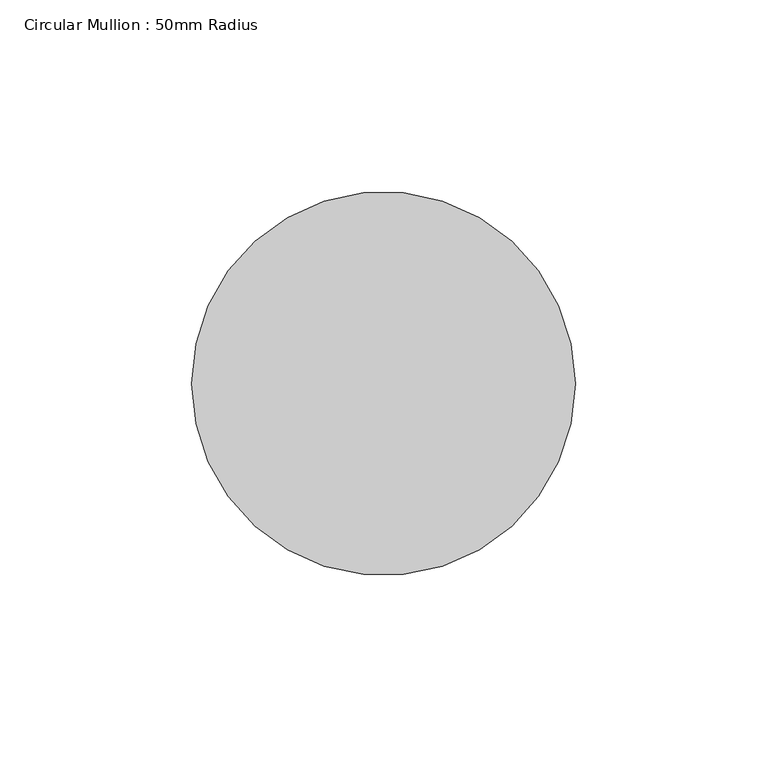
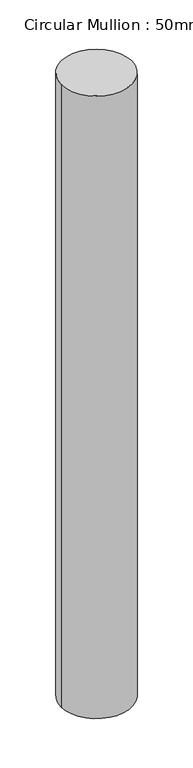
"""IFC4 building model written with IfcOpenShell, lengths in millimetres: member geometry, Circular Mullion : 50mm Radius."""

import ifcopenshell
import ifcopenshell.guid

model = None  # the IFC model being written
_history = None  # IfcOwnerHistory: only IFC2X3 demands one
_inside = {}  # id of a spatial element -> (the spatial element, [elements in it])
_under = {}  # id of a project, library or spatial element -> (it, [spatial elements below it])
_declared = {}  # id of a project -> (the project, [libraries it declares])
_typed = {}  # id of a type object -> (the type object, [elements of that type])
_made_of = {}  # id of a material, layer set ... -> (it, [elements and type objects made of it])


def new_model(schema):
    """Start an empty IFC model of exactly this schema.

    Asked for "IFC4X3", IfcOpenShell would pick the latest addendum, in which some entities
    have other attributes; the version numbers below select the first issue.
    IFC2X3 requires an IfcOwnerHistory on every rooted entity: one is made here for all.
    """
    global model, _history
    if schema == "IFC4X3":
        model = ifcopenshell.file(schema_version=(4, 3, 0, 0))
    else:
        model = ifcopenshell.file(schema=schema)
    _inside.clear()
    _under.clear()
    _declared.clear()
    _typed.clear()
    _made_of.clear()
    _history = None
    if model.schema == "IFC2X3":
        org = make("IfcOrganization", Name="unknown")
        user = make(
            "IfcPersonAndOrganization",
            ThePerson=make("IfcPerson", FamilyName="unknown"),
            TheOrganization=org,
        )
        app = make(
            "IfcApplication",
            ApplicationDeveloper=org,
            Version="unknown",
            ApplicationFullName="unknown",
            ApplicationIdentifier="unknown",
        )
        _history = make(
            "IfcOwnerHistory",
            OwningUser=user,
            OwningApplication=app,
            ChangeAction="ADDED",
            CreationDate=0,
        )
    return model


def make(cls, **values):
    """One entity of the class cls with the attributes given. An attribute that is None is left unset."""
    return model.create_entity(
        cls, **{name: value for name, value in values.items() if value is not None}
    )


def rooted(cls, **values):
    """An entity with a GlobalId (a new one), such as an element, a storey or a relation."""
    return make(cls, GlobalId=ifcopenshell.guid.new(), OwnerHistory=_history, **values)


def si_unit(unit_type, name, prefix=None):
    """IfcSIUnit, for example si_unit("LENGTHUNIT", "METRE", prefix="MILLI")."""
    return make("IfcSIUnit", UnitType=unit_type, Prefix=prefix, Name=name)


def assignment(units):
    """IfcUnitAssignment: the units of a project."""
    return None if units is None else make("IfcUnitAssignment", Units=units)


def point(xyz):
    """IfcCartesianPoint."""
    return None if xyz is None else make("IfcCartesianPoint", Coordinates=xyz)


def direction(xyz):
    """IfcDirection."""
    return None if xyz is None else make("IfcDirection", DirectionRatios=xyz)


def frame(location, z_axis=None, x_axis=None):
    """IfcAxis2Placement3D, a coordinate frame: its origin and axes. An axis left out is left unset."""
    return make(
        "IfcAxis2Placement3D",
        Location=point(location),
        Axis=direction(z_axis),
        RefDirection=direction(x_axis),
    )


def frame_2d(location, x_axis=None):
    """IfcAxis2Placement2D, a coordinate frame in the plane: its origin and x axis."""
    return make(
        "IfcAxis2Placement2D", Location=point(location), RefDirection=direction(x_axis)
    )


def origin():
    """The frame at (0, 0, 0) with its axes left unset."""
    return frame((0.0, 0.0, 0.0))


def origin_2d():
    """The frame at (0, 0) in the plane with its x axis left unset."""
    return frame_2d((0.0, 0.0))


def place(relative_to, where):
    """IfcLocalPlacement: puts the frame where relative to a parent placement (None: the world)."""
    return make(
        "IfcLocalPlacement", PlacementRelTo=relative_to, RelativePlacement=where
    )


def context(
    kind, dimensions, precision=None, world=None, true_north=None, identifier=None
):
    """IfcGeometricRepresentationContext, for example the 3D "Model" context."""
    return make(
        "IfcGeometricRepresentationContext",
        ContextIdentifier=identifier,
        ContextType=kind,
        CoordinateSpaceDimension=dimensions,
        Precision=precision,
        WorldCoordinateSystem=world,
        TrueNorth=true_north,
    )


def project(units=None, contexts=None):
    """IfcProject with its units and contexts."""
    return rooted(
        "IfcProject",
        Name="project",
        RepresentationContexts=contexts,
        UnitsInContext=assignment(units),
    )


def spatial(cls, under=None, at=None, **own):
    """A site, building, storey or space (cls), placed at a placement, below another one or the project."""
    s = rooted(cls, ObjectPlacement=at, **own)
    if under is not None:
        _under.setdefault(under.id(), (under, []))[1].append(s)
    return s


def circle_curve(where, radius):
    """IfcCircle in the frame where."""
    return make("IfcCircle", Position=where, Radius=radius)


def trimmed(basis, trim1, trim2, sense, master):
    """IfcTrimmedCurve: the piece of a basis curve between two trims."""
    return make(
        "IfcTrimmedCurve",
        BasisCurve=basis,
        Trim1=trim1,
        Trim2=trim2,
        SenseAgreement=sense,
        MasterRepresentation=master,
    )


def segment(curve, same_sense, transition):
    """IfcCompositeCurveSegment."""
    return make(
        "IfcCompositeCurveSegment",
        Transition=transition,
        SameSense=same_sense,
        ParentCurve=curve,
    )


def composite_curve(segments, self_intersect=None):
    """IfcCompositeCurve: segments joined end to end."""
    return make("IfcCompositeCurve", Segments=segments, SelfIntersect=self_intersect)


def outline(outer, holes=None, kind="AREA"):
    """IfcArbitraryClosedProfileDef: a profile drawn as a closed curve; with holes, ...WithVoids."""
    if holes is None:
        return make("IfcArbitraryClosedProfileDef", ProfileType=kind, OuterCurve=outer)
    return make(
        "IfcArbitraryProfileDefWithVoids",
        ProfileType=kind,
        OuterCurve=outer,
        InnerCurves=holes,
    )


def extrude(swept, where, along, depth):
    """IfcExtrudedAreaSolid: the profile swept, set in the frame where, extruded along a direction by depth."""
    return make(
        "IfcExtrudedAreaSolid",
        SweptArea=swept,
        Position=where,
        ExtrudedDirection=direction(along),
        Depth=depth,
    )


def shape(context_of_items, identifier, shape_type, items):
    """IfcShapeRepresentation: the items that make up one representation, for example the "Body"."""
    return make(
        "IfcShapeRepresentation",
        ContextOfItems=context_of_items,
        RepresentationIdentifier=identifier,
        RepresentationType=shape_type,
        Items=items,
    )


def source(mapping_origin, context_of_items, identifier, shape_type, items):
    """IfcRepresentationMap: a shape defined once, which mapped items show again and again."""
    return make(
        "IfcRepresentationMap",
        MappingOrigin=mapping_origin,
        MappedRepresentation=shape(context_of_items, identifier, shape_type, items),
    )


def transform(
    local_origin,
    x_axis=None,
    y_axis=None,
    z_axis=None,
    scale=None,
    scale2=None,
    scale3=None,
    uniform=True,
):
    """IfcCartesianTransformationOperator3D, or its non-uniform kind. x_axis, y_axis, z_axis: its Axis1, 2, 3."""
    if uniform:
        return make(
            "IfcCartesianTransformationOperator3D",
            Axis1=direction(x_axis),
            Axis2=direction(y_axis),
            LocalOrigin=point(local_origin),
            Scale=scale,
            Axis3=direction(z_axis),
        )
    return make(
        "IfcCartesianTransformationOperator3DnonUniform",
        Axis1=direction(x_axis),
        Axis2=direction(y_axis),
        LocalOrigin=point(local_origin),
        Scale=scale,
        Axis3=direction(z_axis),
        Scale2=scale2,
        Scale3=scale3,
    )


def mapped(mapping_source, mapping_target):
    """IfcMappedItem: shows the shape of a source again, moved by a transform."""
    return make(
        "IfcMappedItem", MappingSource=mapping_source, MappingTarget=mapping_target
    )


def made_of(thing, what):
    """Note that an element or type object is made of a material, layer set ...; save() writes the relation."""
    if what is not None:
        _made_of.setdefault(what.id(), (what, []))[1].append(thing)
    return thing


def element(
    cls,
    number,
    at=None,
    inside=None,
    cuts=None,
    type_object=None,
    material=None,
    context=None,
    identifier="Body",
    shape_type=None,
    held_by="IfcProductDefinitionShape",
    body=None,
    shapes=None,
    **own,
):
    """One element of the class cls, such as IfcWall. Its Tag is "e" and its number.

    at: its placement. inside: the storey or other place that contains it. cuts: it is an
    opening in that element (IfcRelVoidsElement). A single representation is given by context,
    identifier, shape_type and body (its items); several are given by shapes. held_by: the class
    of the entity that holds the representations. save() writes the other relations.
    """
    e = rooted(cls, Tag="e%d" % number, ObjectPlacement=at, **own)
    if body is not None:
        shapes = [shape(context, identifier, shape_type, body)]
    if shapes is not None:
        e.Representation = make(held_by, Representations=shapes)
    if inside is not None:
        _inside.setdefault(inside.id(), (inside, []))[1].append(e)
    if cuts is not None:
        rooted(
            "IfcRelVoidsElement", RelatingBuildingElement=cuts, RelatedOpeningElement=e
        )
    if type_object is not None:
        _typed.setdefault(type_object.id(), (type_object, []))[1].append(e)
    return made_of(e, material)


def aggregate(whole, parts):
    """IfcRelAggregates: a whole, such as a stair, and the parts it consists of."""
    return rooted("IfcRelAggregates", RelatingObject=whole, RelatedObjects=parts)


def save(model, path):
    """Write the relations noted so far, then the file.

    IfcRelAggregates (storeys below a building ...), IfcRelContainedInSpatialStructure (elements
    in a storey), IfcRelDefinesByType, IfcRelAssociatesMaterial and IfcRelDeclares: one each for
    every whole, place, type object, material and project.
    """
    for whole, parts in _under.values():
        aggregate(whole, parts)
    for where, things in _inside.values():
        rooted(
            "IfcRelContainedInSpatialStructure",
            RelatedElements=things,
            RelatingStructure=where,
        )
    for kind, things in _typed.values():
        rooted("IfcRelDefinesByType", RelatedObjects=things, RelatingType=kind)
    for what, things in _made_of.values():
        rooted("IfcRelAssociatesMaterial", RelatedObjects=things, RelatingMaterial=what)
    for by, libraries in _declared.values():
        rooted("IfcRelDeclares", RelatingContext=by, RelatedDefinitions=libraries)
    model.write(path)


def circular_mullion_50mm_radius_91c7cd3c(model_context):
    return source(origin(), model_context, "Body", "SweptSolid", [
        extrude(outline(composite_curve([segment(trimmed(circle_curve(origin_2d(), 50.0), [point((50.0, 0.0))], [point((-50.0, 0.0))], False, "CARTESIAN"), True, "CONTINUOUS"), segment(trimmed(circle_curve(origin_2d(), 50.0), [point((-50.0, 0.0))], [point((50.0, 0.0))], False, "CARTESIAN"), True, "CONTINUOUS")], self_intersect=False)), frame((0.0, 0.0, -932.67538), z_axis=(0.0, 0.0, 1.0), x_axis=(1.0, 0.0, 0.0)), (0.0, 0.0, 1.0), 932.67538),
    ])


if __name__ == "__main__":
    model = new_model("IFC4")
    model_context = context("Model", 3, world=origin())
    ifc_project = project(units=[si_unit("LENGTHUNIT", "METRE", prefix="MILLI")], contexts=[model_context])
    site = spatial("IfcSite", under=ifc_project)
    building = spatial("IfcBuilding", under=site)
    placement = place(None, origin())
    circular_mullion_50mm_radius_shape = circular_mullion_50mm_radius_91c7cd3c(model_context)
    element("IfcMember", 1, ObjectType="Circular Mullion : 50mm Radius", at=placement, inside=building, context=model_context, shape_type="MappedRepresentation", body=[
        mapped(circular_mullion_50mm_radius_shape, transform((0.0, 0.0, 0.0), x_axis=(1.0, 0.0, 0.0), y_axis=(0.0, 1.0, 0.0), z_axis=(0.0, 0.0, 1.0))),
    ])
    save(model, "model.ifc")

# Revit data of these elements
# Type "Circular Mullion : 50mm Radius"
#   built-in parameter 1007350 = 0.164042 (stored number, unit not read)
# Element 1 (IfcMember, "Circular Mullion : 50mm Radius")
#   Materials on its faces: "Aluminium"
# Materials
#   "Aluminium": class "Metal", colour RGB 247 247 247, transparency 0, Description = "Aluminium 6061", Cost = 0
